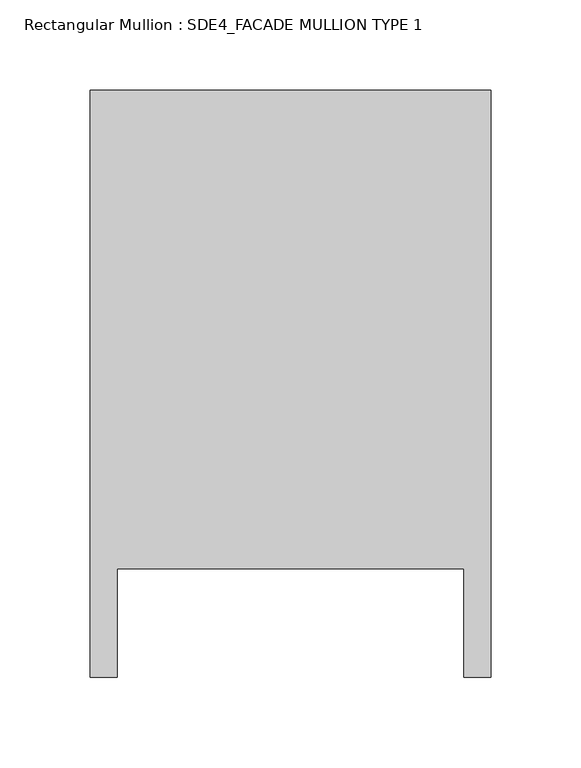
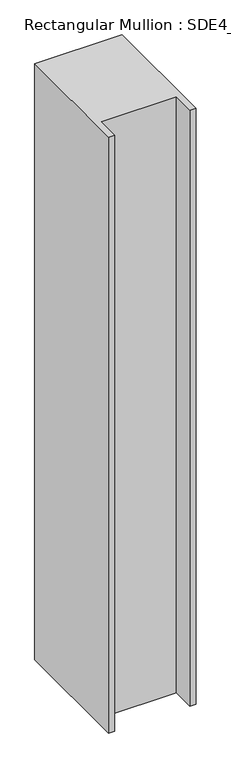
"""IFC4 building model written with IfcOpenShell, lengths in millimetres: member geometry, Rectangular Mullion : SDE4_FACADE MULLION TYPE 1."""

import ifcopenshell
import ifcopenshell.guid

model = None  # the IFC model being written
_history = None  # IfcOwnerHistory: only IFC2X3 demands one
_inside = {}  # id of a spatial element -> (the spatial element, [elements in it])
_under = {}  # id of a project, library or spatial element -> (it, [spatial elements below it])
_declared = {}  # id of a project -> (the project, [libraries it declares])
_typed = {}  # id of a type object -> (the type object, [elements of that type])
_made_of = {}  # id of a material, layer set ... -> (it, [elements and type objects made of it])


def new_model(schema):
    """Start an empty IFC model of exactly this schema.

    Asked for "IFC4X3", IfcOpenShell would pick the latest addendum, in which some entities
    have other attributes; the version numbers below select the first issue.
    IFC2X3 requires an IfcOwnerHistory on every rooted entity: one is made here for all.
    """
    global model, _history
    if schema == "IFC4X3":
        model = ifcopenshell.file(schema_version=(4, 3, 0, 0))
    else:
        model = ifcopenshell.file(schema=schema)
    _inside.clear()
    _under.clear()
    _declared.clear()
    _typed.clear()
    _made_of.clear()
    _history = None
    if model.schema == "IFC2X3":
        org = make("IfcOrganization", Name="unknown")
        user = make(
            "IfcPersonAndOrganization",
            ThePerson=make("IfcPerson", FamilyName="unknown"),
            TheOrganization=org,
        )
        app = make(
            "IfcApplication",
            ApplicationDeveloper=org,
            Version="unknown",
            ApplicationFullName="unknown",
            ApplicationIdentifier="unknown",
        )
        _history = make(
            "IfcOwnerHistory",
            OwningUser=user,
            OwningApplication=app,
            ChangeAction="ADDED",
            CreationDate=0,
        )
    return model


def make(cls, **values):
    """One entity of the class cls with the attributes given. An attribute that is None is left unset."""
    return model.create_entity(
        cls, **{name: value for name, value in values.items() if value is not None}
    )


def rooted(cls, **values):
    """An entity with a GlobalId (a new one), such as an element, a storey or a relation."""
    return make(cls, GlobalId=ifcopenshell.guid.new(), OwnerHistory=_history, **values)


def si_unit(unit_type, name, prefix=None):
    """IfcSIUnit, for example si_unit("LENGTHUNIT", "METRE", prefix="MILLI")."""
    return make("IfcSIUnit", UnitType=unit_type, Prefix=prefix, Name=name)


def assignment(units):
    """IfcUnitAssignment: the units of a project."""
    return None if units is None else make("IfcUnitAssignment", Units=units)


def point(xyz):
    """IfcCartesianPoint."""
    return None if xyz is None else make("IfcCartesianPoint", Coordinates=xyz)


def direction(xyz):
    """IfcDirection."""
    return None if xyz is None else make("IfcDirection", DirectionRatios=xyz)


def frame(location, z_axis=None, x_axis=None):
    """IfcAxis2Placement3D, a coordinate frame: its origin and axes. An axis left out is left unset."""
    return make(
        "IfcAxis2Placement3D",
        Location=point(location),
        Axis=direction(z_axis),
        RefDirection=direction(x_axis),
    )


def origin():
    """The frame at (0, 0, 0) with its axes left unset."""
    return frame((0.0, 0.0, 0.0))


def place(relative_to, where):
    """IfcLocalPlacement: puts the frame where relative to a parent placement (None: the world)."""
    return make(
        "IfcLocalPlacement", PlacementRelTo=relative_to, RelativePlacement=where
    )


def context(
    kind, dimensions, precision=None, world=None, true_north=None, identifier=None
):
    """IfcGeometricRepresentationContext, for example the 3D "Model" context."""
    return make(
        "IfcGeometricRepresentationContext",
        ContextIdentifier=identifier,
        ContextType=kind,
        CoordinateSpaceDimension=dimensions,
        Precision=precision,
        WorldCoordinateSystem=world,
        TrueNorth=true_north,
    )


def project(units=None, contexts=None):
    """IfcProject with its units and contexts."""
    return rooted(
        "IfcProject",
        Name="project",
        RepresentationContexts=contexts,
        UnitsInContext=assignment(units),
    )


def spatial(cls, under=None, at=None, **own):
    """A site, building, storey or space (cls), placed at a placement, below another one or the project."""
    s = rooted(cls, ObjectPlacement=at, **own)
    if under is not None:
        _under.setdefault(under.id(), (under, []))[1].append(s)
    return s


def polyline(points):
    """IfcPolyline through the points."""
    return make("IfcPolyline", Points=[point(p) for p in points])


def outline(outer, holes=None, kind="AREA"):
    """IfcArbitraryClosedProfileDef: a profile drawn as a closed curve; with holes, ...WithVoids."""
    if holes is None:
        return make("IfcArbitraryClosedProfileDef", ProfileType=kind, OuterCurve=outer)
    return make(
        "IfcArbitraryProfileDefWithVoids",
        ProfileType=kind,
        OuterCurve=outer,
        InnerCurves=holes,
    )


def extrude(swept, where, along, depth):
    """IfcExtrudedAreaSolid: the profile swept, set in the frame where, extruded along a direction by depth."""
    return make(
        "IfcExtrudedAreaSolid",
        SweptArea=swept,
        Position=where,
        ExtrudedDirection=direction(along),
        Depth=depth,
    )


def shape(context_of_items, identifier, shape_type, items):
    """IfcShapeRepresentation: the items that make up one representation, for example the "Body"."""
    return make(
        "IfcShapeRepresentation",
        ContextOfItems=context_of_items,
        RepresentationIdentifier=identifier,
        RepresentationType=shape_type,
        Items=items,
    )


def source(mapping_origin, context_of_items, identifier, shape_type, items):
    """IfcRepresentationMap: a shape defined once, which mapped items show again and again."""
    return make(
        "IfcRepresentationMap",
        MappingOrigin=mapping_origin,
        MappedRepresentation=shape(context_of_items, identifier, shape_type, items),
    )


def transform(
    local_origin,
    x_axis=None,
    y_axis=None,
    z_axis=None,
    scale=None,
    scale2=None,
    scale3=None,
    uniform=True,
):
    """IfcCartesianTransformationOperator3D, or its non-uniform kind. x_axis, y_axis, z_axis: its Axis1, 2, 3."""
    if uniform:
        return make(
            "IfcCartesianTransformationOperator3D",
            Axis1=direction(x_axis),
            Axis2=direction(y_axis),
            LocalOrigin=point(local_origin),
            Scale=scale,
            Axis3=direction(z_axis),
        )
    return make(
        "IfcCartesianTransformationOperator3DnonUniform",
        Axis1=direction(x_axis),
        Axis2=direction(y_axis),
        LocalOrigin=point(local_origin),
        Scale=scale,
        Axis3=direction(z_axis),
        Scale2=scale2,
        Scale3=scale3,
    )


def mapped(mapping_source, mapping_target):
    """IfcMappedItem: shows the shape of a source again, moved by a transform."""
    return make(
        "IfcMappedItem", MappingSource=mapping_source, MappingTarget=mapping_target
    )


def made_of(thing, what):
    """Note that an element or type object is made of a material, layer set ...; save() writes the relation."""
    if what is not None:
        _made_of.setdefault(what.id(), (what, []))[1].append(thing)
    return thing


def element(
    cls,
    number,
    at=None,
    inside=None,
    cuts=None,
    type_object=None,
    material=None,
    context=None,
    identifier="Body",
    shape_type=None,
    held_by="IfcProductDefinitionShape",
    body=None,
    shapes=None,
    **own,
):
    """One element of the class cls, such as IfcWall. Its Tag is "e" and its number.

    at: its placement. inside: the storey or other place that contains it. cuts: it is an
    opening in that element (IfcRelVoidsElement). A single representation is given by context,
    identifier, shape_type and body (its items); several are given by shapes. held_by: the class
    of the entity that holds the representations. save() writes the other relations.
    """
    e = rooted(cls, Tag="e%d" % number, ObjectPlacement=at, **own)
    if body is not None:
        shapes = [shape(context, identifier, shape_type, body)]
    if shapes is not None:
        e.Representation = make(held_by, Representations=shapes)
    if inside is not None:
        _inside.setdefault(inside.id(), (inside, []))[1].append(e)
    if cuts is not None:
        rooted(
            "IfcRelVoidsElement", RelatingBuildingElement=cuts, RelatedOpeningElement=e
        )
    if type_object is not None:
        _typed.setdefault(type_object.id(), (type_object, []))[1].append(e)
    return made_of(e, material)


def aggregate(whole, parts):
    """IfcRelAggregates: a whole, such as a stair, and the parts it consists of."""
    return rooted("IfcRelAggregates", RelatingObject=whole, RelatedObjects=parts)


def save(model, path):
    """Write the relations noted so far, then the file.

    IfcRelAggregates (storeys below a building ...), IfcRelContainedInSpatialStructure (elements
    in a storey), IfcRelDefinesByType, IfcRelAssociatesMaterial and IfcRelDeclares: one each for
    every whole, place, type object, material and project.
    """
    for whole, parts in _under.values():
        aggregate(whole, parts)
    for where, things in _inside.values():
        rooted(
            "IfcRelContainedInSpatialStructure",
            RelatedElements=things,
            RelatingStructure=where,
        )
    for kind, things in _typed.values():
        rooted("IfcRelDefinesByType", RelatedObjects=things, RelatingType=kind)
    for what, things in _made_of.values():
        rooted("IfcRelAssociatesMaterial", RelatedObjects=things, RelatingMaterial=what)
    for by, libraries in _declared.values():
        rooted("IfcRelDeclares", RelatingContext=by, RelatedDefinitions=libraries)
    model.write(path)


def rectangular_mullion_sde4_facade_mullion_type_1_e72fc73b(model_context):
    return source(origin(), model_context, "Body", "SweptSolid", [
        extrude(outline(polyline([(111.0, 132.5), (111.0, -192.5), (96.0, -192.5), (96.0, -132.5), (-96.0, -132.5), (-96.0, -192.5), (-111.0, -192.5), (-111.0, 132.5), (111.0, 132.5)])), frame((0.0, 0.0, -1600.0), z_axis=(0.0, 0.0, 1.0), x_axis=(1.0, 0.0, 0.0)), (0.0, 0.0, 1.0), 1600.0),
    ])


if __name__ == "__main__":
    model = new_model("IFC4")
    model_context = context("Model", 3, world=origin())
    ifc_project = project(units=[si_unit("LENGTHUNIT", "METRE", prefix="MILLI")], contexts=[model_context])
    site = spatial("IfcSite", under=ifc_project)
    building = spatial("IfcBuilding", under=site)
    placement = place(None, origin())
    rectangular_mullion_sde4_facade_mullion_type_1_shape = rectangular_mullion_sde4_facade_mullion_type_1_e72fc73b(model_context)
    element("IfcMember", 1, ObjectType="Rectangular Mullion : SDE4_FACADE MULLION TYPE 1", at=placement, inside=building, context=model_context, shape_type="MappedRepresentation", body=[
        mapped(rectangular_mullion_sde4_facade_mullion_type_1_shape, transform((0.0, 0.0, 0.0), x_axis=(1.0, 0.0, 0.0), y_axis=(0.0, 1.0, 0.0), z_axis=(0.0, 0.0, 1.0))),
    ])
    save(model, "model.ifc")

# Revit data of these elements
# Type "Rectangular Mullion : SDE4_FACADE MULLION TYPE 1"
#   built-in parameter 1007322 = 0.869423 (stored number, unit not read)
#   built-in parameter 1007321 = 0.364173 (stored number, unit not read)
#   built-in parameter 1007320 = 0.364173 (stored number, unit not read)
